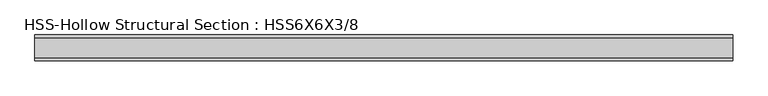
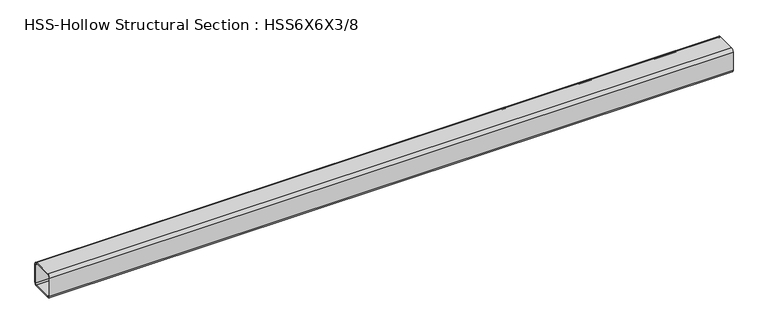
"""IFC4 building model written with IfcOpenShell, lengths in millimetres: member geometry, HSS-Hollow Structural Section : HSS6X6X3/8."""

import ifcopenshell
import ifcopenshell.guid

model = None  # the IFC model being written
_history = None  # IfcOwnerHistory: only IFC2X3 demands one
_inside = {}  # id of a spatial element -> (the spatial element, [elements in it])
_under = {}  # id of a project, library or spatial element -> (it, [spatial elements below it])
_declared = {}  # id of a project -> (the project, [libraries it declares])
_typed = {}  # id of a type object -> (the type object, [elements of that type])
_made_of = {}  # id of a material, layer set ... -> (it, [elements and type objects made of it])


def new_model(schema):
    """Start an empty IFC model of exactly this schema.

    Asked for "IFC4X3", IfcOpenShell would pick the latest addendum, in which some entities
    have other attributes; the version numbers below select the first issue.
    IFC2X3 requires an IfcOwnerHistory on every rooted entity: one is made here for all.
    """
    global model, _history
    if schema == "IFC4X3":
        model = ifcopenshell.file(schema_version=(4, 3, 0, 0))
    else:
        model = ifcopenshell.file(schema=schema)
    _inside.clear()
    _under.clear()
    _declared.clear()
    _typed.clear()
    _made_of.clear()
    _history = None
    if model.schema == "IFC2X3":
        org = make("IfcOrganization", Name="unknown")
        user = make(
            "IfcPersonAndOrganization",
            ThePerson=make("IfcPerson", FamilyName="unknown"),
            TheOrganization=org,
        )
        app = make(
            "IfcApplication",
            ApplicationDeveloper=org,
            Version="unknown",
            ApplicationFullName="unknown",
            ApplicationIdentifier="unknown",
        )
        _history = make(
            "IfcOwnerHistory",
            OwningUser=user,
            OwningApplication=app,
            ChangeAction="ADDED",
            CreationDate=0,
        )
    return model


def make(cls, **values):
    """One entity of the class cls with the attributes given. An attribute that is None is left unset."""
    return model.create_entity(
        cls, **{name: value for name, value in values.items() if value is not None}
    )


def rooted(cls, **values):
    """An entity with a GlobalId (a new one), such as an element, a storey or a relation."""
    return make(cls, GlobalId=ifcopenshell.guid.new(), OwnerHistory=_history, **values)


def si_unit(unit_type, name, prefix=None):
    """IfcSIUnit, for example si_unit("LENGTHUNIT", "METRE", prefix="MILLI")."""
    return make("IfcSIUnit", UnitType=unit_type, Prefix=prefix, Name=name)


def assignment(units):
    """IfcUnitAssignment: the units of a project."""
    return None if units is None else make("IfcUnitAssignment", Units=units)


def point(xyz):
    """IfcCartesianPoint."""
    return None if xyz is None else make("IfcCartesianPoint", Coordinates=xyz)


def direction(xyz):
    """IfcDirection."""
    return None if xyz is None else make("IfcDirection", DirectionRatios=xyz)


def frame(location, z_axis=None, x_axis=None):
    """IfcAxis2Placement3D, a coordinate frame: its origin and axes. An axis left out is left unset."""
    return make(
        "IfcAxis2Placement3D",
        Location=point(location),
        Axis=direction(z_axis),
        RefDirection=direction(x_axis),
    )


def frame_2d(location, x_axis=None):
    """IfcAxis2Placement2D, a coordinate frame in the plane: its origin and x axis."""
    return make(
        "IfcAxis2Placement2D", Location=point(location), RefDirection=direction(x_axis)
    )


def origin():
    """The frame at (0, 0, 0) with its axes left unset."""
    return frame((0.0, 0.0, 0.0))


def place(relative_to, where):
    """IfcLocalPlacement: puts the frame where relative to a parent placement (None: the world)."""
    return make(
        "IfcLocalPlacement", PlacementRelTo=relative_to, RelativePlacement=where
    )


def context(
    kind, dimensions, precision=None, world=None, true_north=None, identifier=None
):
    """IfcGeometricRepresentationContext, for example the 3D "Model" context."""
    return make(
        "IfcGeometricRepresentationContext",
        ContextIdentifier=identifier,
        ContextType=kind,
        CoordinateSpaceDimension=dimensions,
        Precision=precision,
        WorldCoordinateSystem=world,
        TrueNorth=true_north,
    )


def project(units=None, contexts=None):
    """IfcProject with its units and contexts."""
    return rooted(
        "IfcProject",
        Name="project",
        RepresentationContexts=contexts,
        UnitsInContext=assignment(units),
    )


def spatial(cls, under=None, at=None, **own):
    """A site, building, storey or space (cls), placed at a placement, below another one or the project."""
    s = rooted(cls, ObjectPlacement=at, **own)
    if under is not None:
        _under.setdefault(under.id(), (under, []))[1].append(s)
    return s


def polyline(points):
    """IfcPolyline through the points."""
    return make("IfcPolyline", Points=[point(p) for p in points])


def circle_curve(where, radius):
    """IfcCircle in the frame where."""
    return make("IfcCircle", Position=where, Radius=radius)


def trimmed(basis, trim1, trim2, sense, master):
    """IfcTrimmedCurve: the piece of a basis curve between two trims."""
    return make(
        "IfcTrimmedCurve",
        BasisCurve=basis,
        Trim1=trim1,
        Trim2=trim2,
        SenseAgreement=sense,
        MasterRepresentation=master,
    )


def segment(curve, same_sense, transition):
    """IfcCompositeCurveSegment."""
    return make(
        "IfcCompositeCurveSegment",
        Transition=transition,
        SameSense=same_sense,
        ParentCurve=curve,
    )


def composite_curve(segments, self_intersect=None):
    """IfcCompositeCurve: segments joined end to end."""
    return make("IfcCompositeCurve", Segments=segments, SelfIntersect=self_intersect)


def outline(outer, holes=None, kind="AREA"):
    """IfcArbitraryClosedProfileDef: a profile drawn as a closed curve; with holes, ...WithVoids."""
    if holes is None:
        return make("IfcArbitraryClosedProfileDef", ProfileType=kind, OuterCurve=outer)
    return make(
        "IfcArbitraryProfileDefWithVoids",
        ProfileType=kind,
        OuterCurve=outer,
        InnerCurves=holes,
    )


def extrude(swept, where, along, depth):
    """IfcExtrudedAreaSolid: the profile swept, set in the frame where, extruded along a direction by depth."""
    return make(
        "IfcExtrudedAreaSolid",
        SweptArea=swept,
        Position=where,
        ExtrudedDirection=direction(along),
        Depth=depth,
    )


def shape(context_of_items, identifier, shape_type, items):
    """IfcShapeRepresentation: the items that make up one representation, for example the "Body"."""
    return make(
        "IfcShapeRepresentation",
        ContextOfItems=context_of_items,
        RepresentationIdentifier=identifier,
        RepresentationType=shape_type,
        Items=items,
    )


def source(mapping_origin, context_of_items, identifier, shape_type, items):
    """IfcRepresentationMap: a shape defined once, which mapped items show again and again."""
    return make(
        "IfcRepresentationMap",
        MappingOrigin=mapping_origin,
        MappedRepresentation=shape(context_of_items, identifier, shape_type, items),
    )


def transform(
    local_origin,
    x_axis=None,
    y_axis=None,
    z_axis=None,
    scale=None,
    scale2=None,
    scale3=None,
    uniform=True,
):
    """IfcCartesianTransformationOperator3D, or its non-uniform kind. x_axis, y_axis, z_axis: its Axis1, 2, 3."""
    if uniform:
        return make(
            "IfcCartesianTransformationOperator3D",
            Axis1=direction(x_axis),
            Axis2=direction(y_axis),
            LocalOrigin=point(local_origin),
            Scale=scale,
            Axis3=direction(z_axis),
        )
    return make(
        "IfcCartesianTransformationOperator3DnonUniform",
        Axis1=direction(x_axis),
        Axis2=direction(y_axis),
        LocalOrigin=point(local_origin),
        Scale=scale,
        Axis3=direction(z_axis),
        Scale2=scale2,
        Scale3=scale3,
    )


def mapped(mapping_source, mapping_target):
    """IfcMappedItem: shows the shape of a source again, moved by a transform."""
    return make(
        "IfcMappedItem", MappingSource=mapping_source, MappingTarget=mapping_target
    )


def made_of(thing, what):
    """Note that an element or type object is made of a material, layer set ...; save() writes the relation."""
    if what is not None:
        _made_of.setdefault(what.id(), (what, []))[1].append(thing)
    return thing


def element(
    cls,
    number,
    at=None,
    inside=None,
    cuts=None,
    type_object=None,
    material=None,
    context=None,
    identifier="Body",
    shape_type=None,
    held_by="IfcProductDefinitionShape",
    body=None,
    shapes=None,
    **own,
):
    """One element of the class cls, such as IfcWall. Its Tag is "e" and its number.

    at: its placement. inside: the storey or other place that contains it. cuts: it is an
    opening in that element (IfcRelVoidsElement). A single representation is given by context,
    identifier, shape_type and body (its items); several are given by shapes. held_by: the class
    of the entity that holds the representations. save() writes the other relations.
    """
    e = rooted(cls, Tag="e%d" % number, ObjectPlacement=at, **own)
    if body is not None:
        shapes = [shape(context, identifier, shape_type, body)]
    if shapes is not None:
        e.Representation = make(held_by, Representations=shapes)
    if inside is not None:
        _inside.setdefault(inside.id(), (inside, []))[1].append(e)
    if cuts is not None:
        rooted(
            "IfcRelVoidsElement", RelatingBuildingElement=cuts, RelatedOpeningElement=e
        )
    if type_object is not None:
        _typed.setdefault(type_object.id(), (type_object, []))[1].append(e)
    return made_of(e, material)


def aggregate(whole, parts):
    """IfcRelAggregates: a whole, such as a stair, and the parts it consists of."""
    return rooted("IfcRelAggregates", RelatingObject=whole, RelatedObjects=parts)


def save(model, path):
    """Write the relations noted so far, then the file.

    IfcRelAggregates (storeys below a building ...), IfcRelContainedInSpatialStructure (elements
    in a storey), IfcRelDefinesByType, IfcRelAssociatesMaterial and IfcRelDeclares: one each for
    every whole, place, type object, material and project.
    """
    for whole, parts in _under.values():
        aggregate(whole, parts)
    for where, things in _inside.values():
        rooted(
            "IfcRelContainedInSpatialStructure",
            RelatedElements=things,
            RelatingStructure=where,
        )
    for kind, things in _typed.values():
        rooted("IfcRelDefinesByType", RelatedObjects=things, RelatingType=kind)
    for what, things in _made_of.values():
        rooted("IfcRelAssociatesMaterial", RelatedObjects=things, RelatingMaterial=what)
    for by, libraries in _declared.values():
        rooted("IfcRelDeclares", RelatingContext=by, RelatedDefinitions=libraries)
    model.write(path)


def hss_hollow_structural_section_hss6x6x3_8_9fe39c4d(model_context):
    return source(origin(), model_context, "Body", "SweptSolid", [
        extrude(outline(composite_curve([segment(polyline([(76.2, 58.4708), (76.2, -58.4708)]), True, "CONTINUOUS"), segment(trimmed(circle_curve(frame_2d((58.4708, -58.4708)), 17.7292), [point((76.2, -58.4708))], [point((58.4708, -76.2))], False, "CARTESIAN"), True, "CONTINUOUS"), segment(polyline([(58.4708, -76.2), (-58.4708, -76.2)]), True, "CONTINUOUS"), segment(trimmed(circle_curve(frame_2d((-58.4708, -58.4708)), 17.7292), [point((-58.4708, -76.2))], [point((-76.2, -58.4708))], False, "CARTESIAN"), True, "CONTINUOUS"), segment(polyline([(-76.2, -58.4708), (-76.2, 58.4708)]), True, "CONTINUOUS"), segment(trimmed(circle_curve(frame_2d((-58.4708, 58.4708)), 17.7292), [point((-76.2, 58.4708))], [point((-58.4708, 76.2))], False, "CARTESIAN"), True, "CONTINUOUS"), segment(polyline([(-58.4708, 76.2), (58.4708, 76.2)]), True, "CONTINUOUS"), segment(trimmed(circle_curve(frame_2d((58.4708, 58.4708)), 17.7292), [point((58.4708, 76.2))], [point((76.2, 58.4708))], False, "CARTESIAN"), True, "CONTINUOUS")], self_intersect=False), holes=[composite_curve([segment(trimmed(circle_curve(frame_2d((-58.4708, 58.4708)), 8.8646), [point((-58.4708, 67.3354))], [point((-67.3354, 58.4708))], True, "CARTESIAN"), True, "CONTINUOUS"), segment(polyline([(-67.3354, 58.4708), (-67.3354, -58.4708)]), True, "CONTINUOUS"), segment(trimmed(circle_curve(frame_2d((-58.4708, -58.4708)), 8.8646), [point((-67.3354, -58.4708))], [point((-58.4708, -67.3354))], True, "CARTESIAN"), True, "CONTINUOUS"), segment(polyline([(-58.4708, -67.3354), (58.4708, -67.3354)]), True, "CONTINUOUS"), segment(trimmed(circle_curve(frame_2d((58.4708, -58.4708)), 8.8646), [point((58.4708, -67.3354))], [point((67.3354, -58.4708))], True, "CARTESIAN"), True, "CONTINUOUS"), segment(polyline([(67.3354, -58.4708), (67.3354, 58.4708)]), True, "CONTINUOUS"), segment(trimmed(circle_curve(frame_2d((58.4708, 58.4708)), 8.8646), [point((67.3354, 58.4708))], [point((58.4708, 67.3354))], True, "CARTESIAN"), True, "CONTINUOUS"), segment(polyline([(58.4708, 67.3354), (-58.4708, 67.3354)]), True, "CONTINUOUS")], self_intersect=False)]), frame((-2038.2688863, 0.0, 0.0), z_axis=(1.0, 0.0, 0.0), x_axis=(0.0, 1.0, 0.0)), (0.0, 0.0, 1.0), 4138.0001242),
    ])


if __name__ == "__main__":
    model = new_model("IFC4")
    model_context = context("Model", 3, world=origin())
    ifc_project = project(units=[si_unit("LENGTHUNIT", "METRE", prefix="MILLI")], contexts=[model_context])
    site = spatial("IfcSite", under=ifc_project)
    building = spatial("IfcBuilding", under=site)
    placement = place(None, origin())
    hss_hollow_structural_section_hss6x6x3_8_shape = hss_hollow_structural_section_hss6x6x3_8_9fe39c4d(model_context)
    element("IfcMember", 1, ObjectType="HSS-Hollow Structural Section : HSS6X6X3/8", at=placement, inside=building, context=model_context, shape_type="MappedRepresentation", body=[
        mapped(hss_hollow_structural_section_hss6x6x3_8_shape, transform((0.0, 0.0, 0.0), x_axis=(1.0, 0.0, 0.0), y_axis=(0.0, 1.0, 0.0), z_axis=(0.0, 0.0, 1.0))),
    ])
    save(model, "model.ifc")

# Revit data of these elements
# Type "HSS-Hollow Structural Section : HSS6X6X3/8"
#   Assembly Code = "B10"
#   Shape = "Square"
#   W = 27.4
#   Ht = 0' - 6"
#   Length [instance default] = 5' - 0"
#   b = 0' - 6"
#   kr = 0' - 0.698"
#   t = 0' - 0.349"
#   A = 0.0526389 SF
#   Structural Material [instance default] = Steel ASTM A500, Grade B, Rectangular and Square
# Element 1 (IfcMember, "HSS-Hollow Structural Section : HSS6X6X3/8")
#   Materials on its faces: "Steel ASTM A500, Grade B, Rectangular and Square"
# Materials
#   "Steel ASTM A500, Grade B, Rectangular and Square": class "Metal", colour RGB 199 199 199, transparency 0, Description = "Carbon steel", Cost = 0
